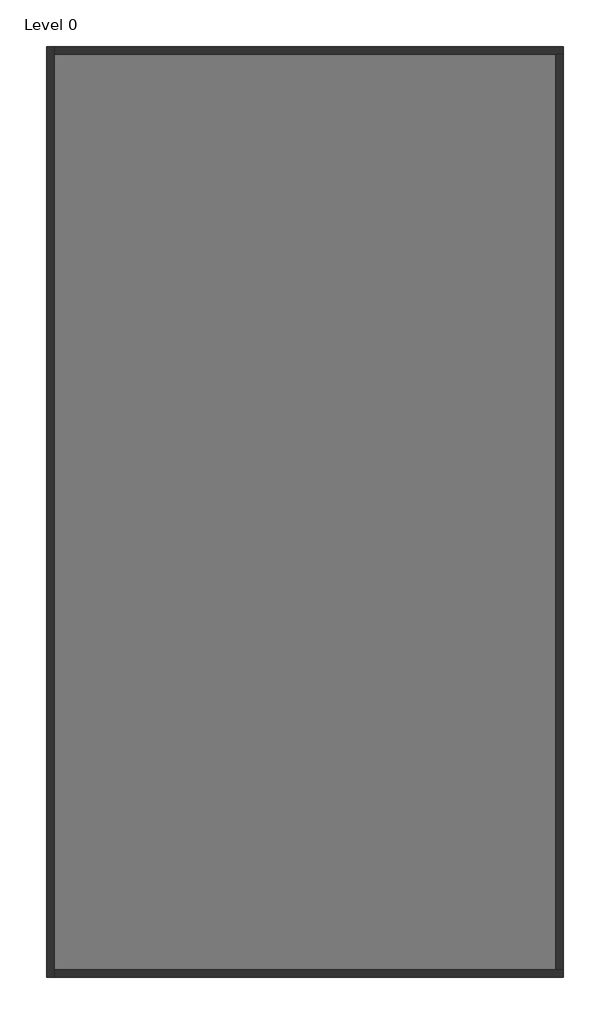
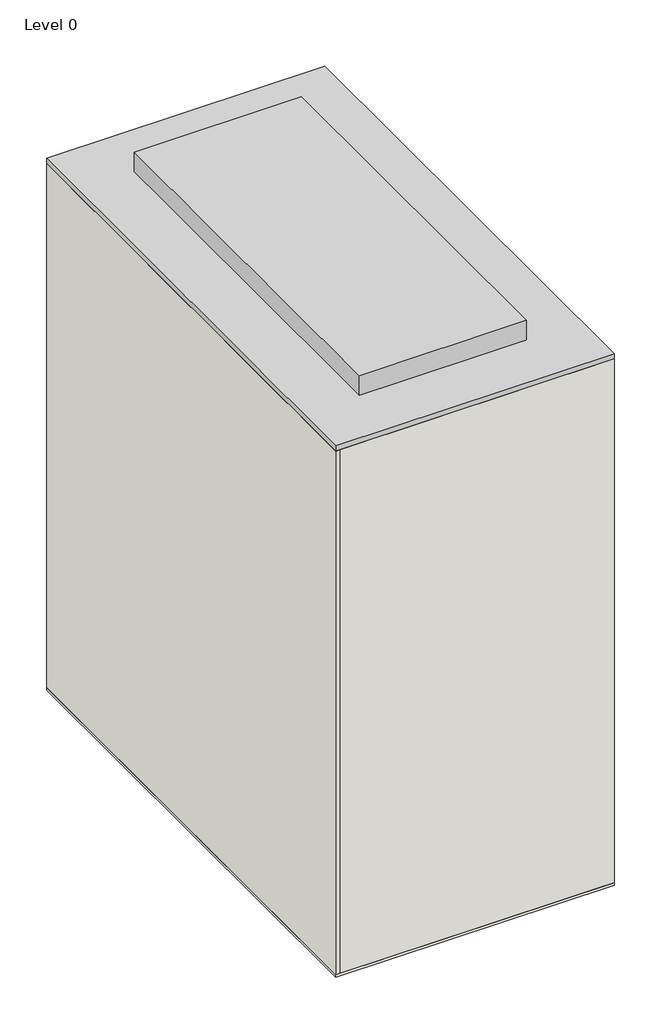
# One storey: 4 walls, 1 proxy, 1 slab.
"""IFC4 building model written with IfcOpenShell, lengths in millimetres."""

from ifc_helpers import new_model, si_unit, frame, origin, origin_with_axes, place, context, project, spatial, polyline, outline, extrude, faceted_brep, element, save

model = new_model("IFC4")

# Units and contexts
model_context = context("Model", 3, world=origin())
ifc_project = project(units=[si_unit("LENGTHUNIT", "METRE", prefix="MILLI")], contexts=[model_context])

# Site, building, storey
site = spatial("IfcSite", under=ifc_project)
building = spatial("IfcBuilding", under=site)
storey = spatial("IfcBuildingStorey", under=building, Name="Level 0", Elevation=100.0)

# Proxy
placement = place(None, origin())
element("IfcBuildingElementProxy", 1, Name="LowUrbanDensityBuilding : LowUrbanDensityBuilding", ObjectType="LowUrbanDensityBuilding : LowUrbanDensityBuilding", at=placement, inside=storey, context=model_context, shape_type="SweptSolid", body=[
    extrude(outline(polyline([(7325.2659446, 3676.2074539), (7325.2659446, -14323.7925461), (-2674.7340554, -14323.7925461), (-2674.7340554, 3676.2074539), (7325.2659446, 3676.2074539)])), origin_with_axes(), (0.0, 0.0, 1.0), 20200.0),
    extrude(outline(polyline([(5325.2659446, 1676.2074539), (5325.2659446, -12323.7925461), (-674.7340554, -12323.7925461), (-674.7340554, 1676.2074539), (5325.2659446, 1676.2074539)])), frame((0.0, 0.0, 20200.0), z_axis=(0.0, 0.0, 1.0), x_axis=(1.0, 0.0, 0.0)), (0.0, 0.0, 1.0), 749.8),
])

# Slab
element("IfcSlab", 2, ObjectType="Floor-Concrete_100Con", at=placement, inside=storey, context=model_context, shape_type="SweptSolid", body=[
    extrude(outline(polyline([(7325.2659446, 3676.2074539), (7325.2659446, -14323.7925461), (-2674.7340554, -14323.7925461), (-2674.7340554, 3676.2074539), (7325.2659446, 3676.2074539)])), origin_with_axes(), (0.0, 0.0, 1.0), 100.0),
])

# Walls
element("IfcWall", 3, ObjectType="Wall-Ext_25Rdr-100Blk-19P", at=placement, inside=storey, context=model_context, shape_type="Brep", body=[
    faceted_brep([(-2674.7340554, 3676.2074539, 100.0), (-2674.7340554, -14323.7925461, 100.0), (-2674.7340554, -14323.7925461, 20000.0), (-2674.7340554, 3676.2074539, 20000.0), (-2530.4340554, 3676.2074539, 100.0), (-2530.4340554, 3676.2074539, 20000.0), (-2530.4340554, 3531.9074539, 20000.0), (-2530.4340554, -14179.4925461, 20000.0), (-2530.4340554, -14323.7925461, 20000.0), (-2530.4340554, -14323.7925461, 100.0), (-2530.4340554, -14179.4925461, 100.0), (-2530.4340554, 3531.9074539, 100.0)], [[[0, 1, 2, 3]], [[4, 5, 6, 7, 8, 9, 10, 11]], [[1, 0, 4, 11, 10, 9]], [[3, 2, 8, 7, 6, 5]], [[2, 1, 9, 8]], [[0, 3, 5, 4]]]),
])
element("IfcWall", 4, ObjectType="Wall-Ext_25Rdr-100Blk-19P", at=placement, inside=storey, context=model_context, shape_type="Brep", body=[
    faceted_brep([(-2530.4340554, -14323.7925461, 100.0), (7325.2659446, -14323.7925461, 100.0), (7325.2659446, -14323.7925461, 20000.0), (-2530.4340554, -14323.7925461, 20000.0), (-2530.4340554, -14179.4925461, 100.0), (-2530.4340554, -14179.4925461, 20000.0), (7180.9659446, -14179.4925461, 20000.0), (7325.2659446, -14179.4925461, 20000.0), (7325.2659446, -14179.4925461, 100.0), (7180.9659446, -14179.4925461, 100.0)], [[[0, 1, 2, 3]], [[4, 5, 6, 7, 8, 9]], [[1, 0, 4, 9, 8]], [[3, 2, 7, 6, 5]], [[0, 3, 5, 4]], [[2, 1, 8, 7]]]),
])
element("IfcWall", 5, ObjectType="Wall-Ext_25Rdr-100Blk-19P", at=placement, inside=storey, context=model_context, shape_type="Brep", body=[
    faceted_brep([(7325.2659446, 3676.2074539, 100.0), (-2530.4340554, 3676.2074539, 100.0), (-2530.4340554, 3676.2074539, 20000.0), (7325.2659446, 3676.2074539, 20000.0), (7325.2659446, 3531.9074539, 100.0), (7325.2659446, 3531.9074539, 20000.0), (7180.9659446, 3531.9074539, 20000.0), (-2530.4340554, 3531.9074539, 20000.0), (-2530.4340554, 3531.9074539, 100.0), (7180.9659446, 3531.9074539, 100.0)], [[[0, 1, 2, 3]], [[4, 5, 6, 7, 8, 9]], [[1, 0, 4, 9, 8]], [[3, 2, 7, 6, 5]], [[2, 1, 8, 7]], [[0, 3, 5, 4]]]),
])
element("IfcWall", 6, ObjectType="Wall-Ext_25Rdr-100Blk-19P", at=placement, inside=storey, context=model_context, shape_type="SweptSolid", body=[
    extrude(outline(polyline([(7325.2659446, 3531.9074539), (7325.2659446, -14179.4925461), (7180.9659446, -14179.4925461), (7180.9659446, 3531.9074539), (7325.2659446, 3531.9074539)])), frame((0.0, 0.0, 100.0), z_axis=(0.0, 0.0, 1.0), x_axis=(1.0, 0.0, 0.0)), (0.0, 0.0, 1.0), 19900.0),
])

save(model, "model.ifc")

# Revit data of these elements
# Project information
#   Project Issue Date = "Issue Date"
#   Project Status = "Project Status"
#   Client Name = "Owner"
#   Project Address = "Enter address here"
#   Project Name = "Project Name"
#   Project Number = "Project Number"
# Type "Floor-Concrete_100Con"
#   Keynote = "E60/130"
#   Function = 0
#   Layers, outside or top first: 100 mm "Concrete" (function 1)
# Type "Wall-Ext_25Rdr-100Blk-19P"
#   Keynote = "F10"
#   Layers, outside or top first: 25.3 mm "Render, Beige, Smooth" (function 5); 100 mm "Concrete Masonry Units _Low Density" (function 1); 19 mm "Plaster" (function 5)
# Element 1 (IfcBuildingElementProxy, "LowUrbanDensityBuilding : LowUrbanDensityBuilding")
#   Phase Created = New Construction
#   Materials on its faces: "Default Form"
# Element 2 (IfcSlab, "Floor-Concrete_100Con")
#   Height Offset From Level = 0 mm
#   Phase Created = New Construction
#   Materials on its faces: "Concrete"
# Element 3 (IfcWall, "Wall-Ext_25Rdr-100Blk-19P")
#   Top Offset = 0 mm
#   Base Offset = 0 mm
#   wall height = 19900 mm
#   Phase Created = New Construction
#   Base Constraint = Level 0
#   Top Constraint = Level 5
#   Materials on its faces: "Render, Beige, Smooth", "Default Wall", "Plaster"
# Elements 4, 5, 6 (IfcWall, "Wall-Ext_25Rdr-100Blk-19P")
#   Top Offset = 0 mm
#   Base Offset = 0 mm
#   wall height = 19900 mm
#   Phase Created = New Construction
#   Base Constraint = Level 0
#   Top Constraint = Level 5
#   Materials on its faces: "Default Wall", "Render, Beige, Smooth", "Plaster"
# Materials
#   "Concrete": class "Concrete", colour RGB 120 120 120, transparency 0, Description = "Portland Cement Concrete", Cost = 0
#   "Render, Beige, Smooth": class "Generic", colour RGB 213 198 180, transparency 0, Description = "physical material", Cost = 0
#   "Concrete Masonry Units _Low Density": class "Masonry", colour RGB 181 181 181, transparency 0, Description = "Concrete masonry units", Cost = 0
#   "Plaster": class "Generic", colour RGB 249 249 249, transparency 0, Description = "Plaster", Cost = 0
#   "Default Form": class "Generic", colour RGB 185 189 196, transparency 0.5, Cost = 0
#   "Default Wall": class "Miscellaneous", colour RGB 128 128 128, transparency 0, Comments = "Rendering appearance not upgraded Rendering appearance not upgraded ", Cost = 0
